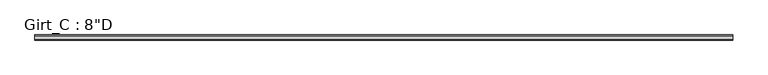
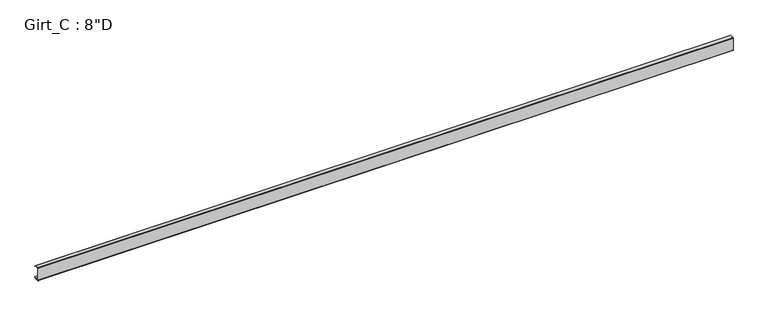
"""IFC4 building model written with IfcOpenShell, lengths in millimetres: beam geometry."""

from ifc_helpers import new_model, si_unit, point, frame, frame_2d, origin, place, context, project, spatial, polyline, circle_curve, trimmed, segment, composite_curve, outline, extrude, source, transform, mapped, element, save


def beam_4ecfc2e4(model_context):
    return source(origin(), model_context, "Body", "SweptSolid", [
        extrude(outline(composite_curve([segment(polyline([(63.5, 101.6), (75.745104, 87.0068534), (73.6169367, 85.221109), (62.204539, 98.821875), (3.3005807, 98.821875)]), True, "CONTINUOUS"), segment(trimmed(circle_curve(frame_2d((3.3741066, 96.8381931)), 1.9850441), [point((3.3005807, 98.821875))], [point((1.3890625, 96.8381931))], True, "CARTESIAN"), True, "CONTINUOUS"), segment(polyline([(1.3890625, 96.8381931), (1.3890625, -96.8389339)]), True, "CONTINUOUS"), segment(trimmed(circle_curve(frame_2d((3.3748024, -96.8389339)), 1.9857399), [point((1.3890625, -96.8389339))], [point((3.2694106, -98.821875))], True, "CARTESIAN"), True, "CONTINUOUS"), segment(polyline([(3.2694106, -98.821875), (62.204539, -98.821875), (73.6169367, -85.221109), (75.745104, -87.0068534), (63.5, -101.6), (3.3734375, -101.6)]), True, "CONTINUOUS"), segment(trimmed(circle_curve(frame_2d((3.3734375, -96.8375)), 4.7625), [point((3.3734375, -101.6))], [point((-1.3890625, -96.8375))], False, "CARTESIAN"), True, "CONTINUOUS"), segment(polyline([(-1.3890625, -96.8375), (-1.3890625, 96.8375)]), True, "CONTINUOUS"), segment(trimmed(circle_curve(frame_2d((3.3734375, 96.8375)), 4.7625), [point((-1.3890625, 96.8375))], [point((3.3734375, 101.6))], False, "CARTESIAN"), True, "CONTINUOUS"), segment(polyline([(3.3734375, 101.6), (63.5, 101.6)]), True, "CONTINUOUS")], self_intersect=False)), frame((-5347.4874, 0.0, 0.0), z_axis=(1.0, 0.0, 0.0), x_axis=(0.0, 1.0, 0.0)), (0.0, 0.0, 1.0), 10539.3998),
    ])


if __name__ == "__main__":
    model = new_model("IFC4")
    model_context = context("Model", 3, world=origin())
    ifc_project = project(units=[si_unit("LENGTHUNIT", "METRE", prefix="MILLI")], contexts=[model_context])
    site = spatial("IfcSite", under=ifc_project)
    building = spatial("IfcBuilding", under=site)
    placement = place(None, origin())
    beam_shape = beam_4ecfc2e4(model_context)
    element("IfcBeam", 1, ObjectType="Girt_C : 8\"D", at=placement, inside=building, context=model_context, shape_type="MappedRepresentation", body=[
        mapped(beam_shape, transform((0.0, 0.0, 0.0), x_axis=(1.0, 0.0, 0.0), y_axis=(0.0, 1.0, 0.0), z_axis=(0.0, 0.0, 1.0))),
    ])
    save(model, "model.ifc")

# Revit data of these elements
# Type "Girt_C : 8\"D"
#   Web_Thickness = 0' - 0 7/64"
#   Length [instance default] = 10' - 0"
#   Leg_1 = 0' - 2 1/2"
#   Height = 0' - 8"
#   Structural Material [instance default] = none
